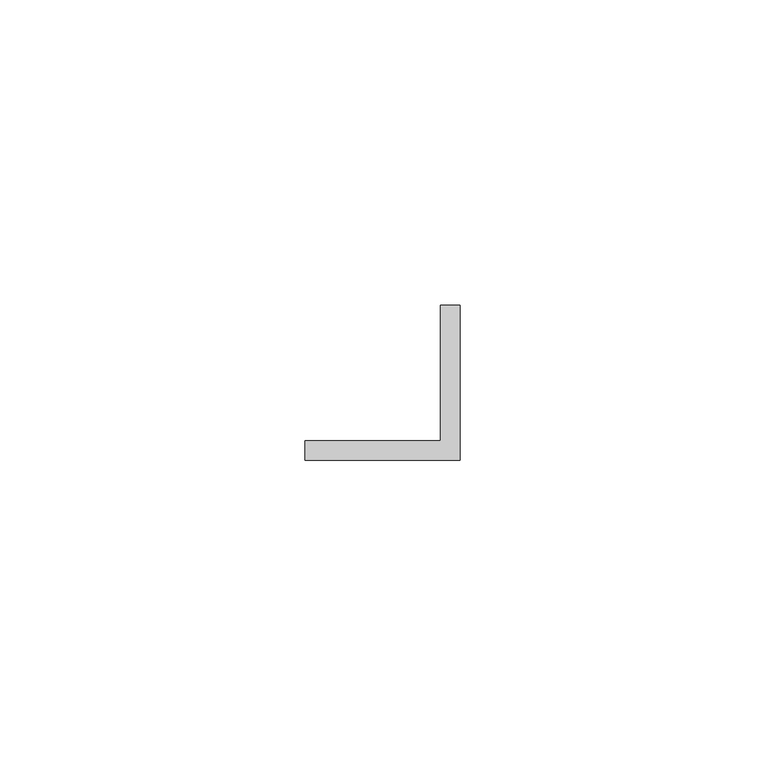
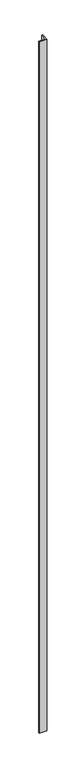
"""IFC4 building model written with IfcOpenShell, lengths in millimetres: proxy geometry, Lower profile:Lower profile:1:Lower profile:1 : Lower profile:Lower profile:300380:301093:Lower profile:1:Lower profile:1 : Lower profile:Lower profile:300380:301093 : Lower profile:Lower profile:1:Lower profile:1 : Lower profile:Lower profile:300380:301093:4 : Lower profile:Lower profile:1:Lower profile:1 : Lower profile:Lower profile:300380:301093:Lower profile:1:Lower profile:1 : Lower profile:Lower profile:300380:301093 : Lower profile:Lower profile:1:Lower profile:1 : Lower profile:Lower profile:300380:301093:300247."""

from ifc_helpers import new_model, si_unit, frame, origin, place, context, project, spatial, polyline, outline, extrude, source, transform, mapped, element, save


def generic_models_ff186d25(model_context):
    return source(origin(), model_context, "Body", "SweptSolid", [
        extrude(outline(polyline([(593738.0867239, -578772.0913841), (593738.0867239, -578797.4913841), (593712.6867239, -578797.4913841), (593712.6867239, -578794.268987), (593734.9117239, -578794.268987), (593734.9117239, -578772.0913841), (593738.0867239, -578772.0913841)])), frame((0.0, 0.0, 14.2875), z_axis=(0.0, 0.0, 1.0), x_axis=(1.0, 0.0, 0.0)), (0.0, 0.0, 1.0), 2438.4),
    ])


if __name__ == "__main__":
    model = new_model("IFC4")
    model_context = context("Model", 3, world=origin())
    ifc_project = project(units=[si_unit("LENGTHUNIT", "METRE", prefix="MILLI")], contexts=[model_context])
    site = spatial("IfcSite", under=ifc_project)
    building = spatial("IfcBuilding", under=site)
    placement = place(None, origin())
    generic_models_shape = generic_models_ff186d25(model_context)
    element("IfcBuildingElementProxy", 1, Name="Lower profile:Lower profile:1:Lower profile:1 : Lower profile:Lower profile:300380:301093:Lower profile:1:Lower profile:1 : Lower profile:Lower profile:300380:301093 : Lower profile:Lower profile:1:Lower profile:1 : Lower profile:Lower profile:300380:301093:4 : Lower profile:Lower profile:1:Lower profile:1 : Lower profile:Lower profile:300380:301093:Lower profile:1:Lower profile:1 : Lower profile:Lower profile:300380:301093 : Lower profile:Lower profile:1:Lower profile:1 : Lower profile:Lower profile:300380:301093:300247", ObjectType="Lower profile:Lower profile:1:Lower profile:1 : Lower profile:Lower profile:300380:301093:Lower profile:1:Lower profile:1 : Lower profile:Lower profile:300380:301093 : Lower profile:Lower profile:1:Lower profile:1 : Lower profile:Lower profile:300380:301093:4 : Lower profile:Lower profile:1:Lower profile:1 : Lower profile:Lower profile:300380:301093:Lower profile:1:Lower profile:1 : Lower profile:Lower profile:300380:301093 : Lower profile:Lower profile:1:Lower profile:1 : Lower profile:Lower profile:300380:301093:300247", at=placement, inside=building, context=model_context, shape_type="MappedRepresentation", body=[
        mapped(generic_models_shape, transform((0.0, 0.0, 0.0), x_axis=(1.0, 0.0, 0.0), y_axis=(0.0, 1.0, 0.0), z_axis=(0.0, 0.0, 1.0))),
    ])
    save(model, "model.ifc")

# Revit data of these elements
# Type "Lower profile:Lower profile:1:Lower profile:1 : Lower profile:Lower profile:300380:301093:Lower profile:1:Lower profile:1 : Lower profile:Lower profile:300380:301093 : Lower profile:Lower profile:1:Lower profile:1 : Lower profile:Lower profile:300380:301093:4 : Lower profile:Lower profile:1:Lower profile:1 : Lower profile:Lower profile:300380:301093:Lower profile:1:Lower profile:1 : Lower profile:Lower profile:300380:301093 : Lower profile:Lower profile:1:Lower profile:1 : Lower profile:Lower profile:300380:301093:300247"
#   NameOverride = "Lower profile:Lower profile:1:Lower profile:1 : Lower profile:Lower profile:300380:301093:Lower profile:1:Lower profile:1 : Lower profile:Lower profile:300380:301093 : Lower profile:Lower profile:1:Lower profile:1 : Lower profile:Lower profile:300380:301093:300247"
#   ObjectTypeOverride = "Lower profile:1:Lower profile:1 : Lower profile:Lower profile:300380:301093 : Lower profile:Lower profile:1:Lower profile:1 : Lower profile:Lower profile:300380:301093"
#   Reference = "Lower profile"
#   Tag = "300247"
# Element 1 (IfcBuildingElementProxy, "Lower profile:Lower profile:1:Lower profile:1 : Lower profile:Lower profile:300380:301093:Lower profile:1:Lower profile:1 : Lower profile:Lower profile:300380:301093 : Lower profile:Lower profile:1:Lower profile:1 : Lower profile:Lower profile:300380:301093:4 : Lower profile:Lower profile:1:Lower profile:1 : Lower profile:Lower profile:300380:301093:Lower profile:1:Lower profile:1 : Lower profile:Lower profile:300380:301093 : Lower profile:Lower profile:1:Lower profile:1 : Lower profile:Lower profile:300380:301093:300247")
#   Materials on its faces: "1\" X 1\" X 1/8\" ALUM. ANGLE"
# Materials
#   "1\" X 1\" X 1/8\" ALUM. ANGLE": class "Metal", colour RGB 244 244 244, transparency 0, Description = "Aluminum 6061", Cost = 0
